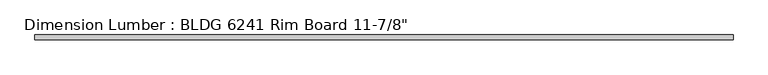
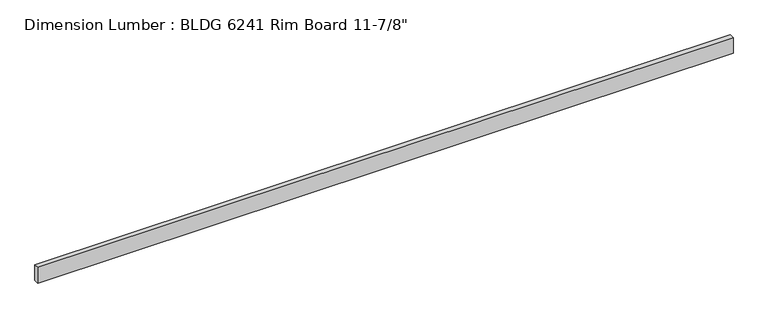
"""IFC4 building model written with IfcOpenShell, lengths in millimetres: beam geometry."""

import ifcopenshell
import ifcopenshell.guid

model = None  # the IFC model being written
_history = None  # IfcOwnerHistory: only IFC2X3 demands one
_inside = {}  # id of a spatial element -> (the spatial element, [elements in it])
_under = {}  # id of a project, library or spatial element -> (it, [spatial elements below it])
_declared = {}  # id of a project -> (the project, [libraries it declares])
_typed = {}  # id of a type object -> (the type object, [elements of that type])
_made_of = {}  # id of a material, layer set ... -> (it, [elements and type objects made of it])


def new_model(schema):
    """Start an empty IFC model of exactly this schema.

    Asked for "IFC4X3", IfcOpenShell would pick the latest addendum, in which some entities
    have other attributes; the version numbers below select the first issue.
    IFC2X3 requires an IfcOwnerHistory on every rooted entity: one is made here for all.
    """
    global model, _history
    if schema == "IFC4X3":
        model = ifcopenshell.file(schema_version=(4, 3, 0, 0))
    else:
        model = ifcopenshell.file(schema=schema)
    _inside.clear()
    _under.clear()
    _declared.clear()
    _typed.clear()
    _made_of.clear()
    _history = None
    if model.schema == "IFC2X3":
        org = make("IfcOrganization", Name="unknown")
        user = make(
            "IfcPersonAndOrganization",
            ThePerson=make("IfcPerson", FamilyName="unknown"),
            TheOrganization=org,
        )
        app = make(
            "IfcApplication",
            ApplicationDeveloper=org,
            Version="unknown",
            ApplicationFullName="unknown",
            ApplicationIdentifier="unknown",
        )
        _history = make(
            "IfcOwnerHistory",
            OwningUser=user,
            OwningApplication=app,
            ChangeAction="ADDED",
            CreationDate=0,
        )
    return model


def make(cls, **values):
    """One entity of the class cls with the attributes given. An attribute that is None is left unset."""
    return model.create_entity(
        cls, **{name: value for name, value in values.items() if value is not None}
    )


def rooted(cls, **values):
    """An entity with a GlobalId (a new one), such as an element, a storey or a relation."""
    return make(cls, GlobalId=ifcopenshell.guid.new(), OwnerHistory=_history, **values)


def si_unit(unit_type, name, prefix=None):
    """IfcSIUnit, for example si_unit("LENGTHUNIT", "METRE", prefix="MILLI")."""
    return make("IfcSIUnit", UnitType=unit_type, Prefix=prefix, Name=name)


def assignment(units):
    """IfcUnitAssignment: the units of a project."""
    return None if units is None else make("IfcUnitAssignment", Units=units)


def point(xyz):
    """IfcCartesianPoint."""
    return None if xyz is None else make("IfcCartesianPoint", Coordinates=xyz)


def direction(xyz):
    """IfcDirection."""
    return None if xyz is None else make("IfcDirection", DirectionRatios=xyz)


def frame(location, z_axis=None, x_axis=None):
    """IfcAxis2Placement3D, a coordinate frame: its origin and axes. An axis left out is left unset."""
    return make(
        "IfcAxis2Placement3D",
        Location=point(location),
        Axis=direction(z_axis),
        RefDirection=direction(x_axis),
    )


def origin():
    """The frame at (0, 0, 0) with its axes left unset."""
    return frame((0.0, 0.0, 0.0))


def place(relative_to, where):
    """IfcLocalPlacement: puts the frame where relative to a parent placement (None: the world)."""
    return make(
        "IfcLocalPlacement", PlacementRelTo=relative_to, RelativePlacement=where
    )


def context(
    kind, dimensions, precision=None, world=None, true_north=None, identifier=None
):
    """IfcGeometricRepresentationContext, for example the 3D "Model" context."""
    return make(
        "IfcGeometricRepresentationContext",
        ContextIdentifier=identifier,
        ContextType=kind,
        CoordinateSpaceDimension=dimensions,
        Precision=precision,
        WorldCoordinateSystem=world,
        TrueNorth=true_north,
    )


def project(units=None, contexts=None):
    """IfcProject with its units and contexts."""
    return rooted(
        "IfcProject",
        Name="project",
        RepresentationContexts=contexts,
        UnitsInContext=assignment(units),
    )


def spatial(cls, under=None, at=None, **own):
    """A site, building, storey or space (cls), placed at a placement, below another one or the project."""
    s = rooted(cls, ObjectPlacement=at, **own)
    if under is not None:
        _under.setdefault(under.id(), (under, []))[1].append(s)
    return s


def polyline(points):
    """IfcPolyline through the points."""
    return make("IfcPolyline", Points=[point(p) for p in points])


def outline(outer, holes=None, kind="AREA"):
    """IfcArbitraryClosedProfileDef: a profile drawn as a closed curve; with holes, ...WithVoids."""
    if holes is None:
        return make("IfcArbitraryClosedProfileDef", ProfileType=kind, OuterCurve=outer)
    return make(
        "IfcArbitraryProfileDefWithVoids",
        ProfileType=kind,
        OuterCurve=outer,
        InnerCurves=holes,
    )


def extrude(swept, where, along, depth):
    """IfcExtrudedAreaSolid: the profile swept, set in the frame where, extruded along a direction by depth."""
    return make(
        "IfcExtrudedAreaSolid",
        SweptArea=swept,
        Position=where,
        ExtrudedDirection=direction(along),
        Depth=depth,
    )


def shape(context_of_items, identifier, shape_type, items):
    """IfcShapeRepresentation: the items that make up one representation, for example the "Body"."""
    return make(
        "IfcShapeRepresentation",
        ContextOfItems=context_of_items,
        RepresentationIdentifier=identifier,
        RepresentationType=shape_type,
        Items=items,
    )


def source(mapping_origin, context_of_items, identifier, shape_type, items):
    """IfcRepresentationMap: a shape defined once, which mapped items show again and again."""
    return make(
        "IfcRepresentationMap",
        MappingOrigin=mapping_origin,
        MappedRepresentation=shape(context_of_items, identifier, shape_type, items),
    )


def transform(
    local_origin,
    x_axis=None,
    y_axis=None,
    z_axis=None,
    scale=None,
    scale2=None,
    scale3=None,
    uniform=True,
):
    """IfcCartesianTransformationOperator3D, or its non-uniform kind. x_axis, y_axis, z_axis: its Axis1, 2, 3."""
    if uniform:
        return make(
            "IfcCartesianTransformationOperator3D",
            Axis1=direction(x_axis),
            Axis2=direction(y_axis),
            LocalOrigin=point(local_origin),
            Scale=scale,
            Axis3=direction(z_axis),
        )
    return make(
        "IfcCartesianTransformationOperator3DnonUniform",
        Axis1=direction(x_axis),
        Axis2=direction(y_axis),
        LocalOrigin=point(local_origin),
        Scale=scale,
        Axis3=direction(z_axis),
        Scale2=scale2,
        Scale3=scale3,
    )


def mapped(mapping_source, mapping_target):
    """IfcMappedItem: shows the shape of a source again, moved by a transform."""
    return make(
        "IfcMappedItem", MappingSource=mapping_source, MappingTarget=mapping_target
    )


def made_of(thing, what):
    """Note that an element or type object is made of a material, layer set ...; save() writes the relation."""
    if what is not None:
        _made_of.setdefault(what.id(), (what, []))[1].append(thing)
    return thing


def element(
    cls,
    number,
    at=None,
    inside=None,
    cuts=None,
    type_object=None,
    material=None,
    context=None,
    identifier="Body",
    shape_type=None,
    held_by="IfcProductDefinitionShape",
    body=None,
    shapes=None,
    **own,
):
    """One element of the class cls, such as IfcWall. Its Tag is "e" and its number.

    at: its placement. inside: the storey or other place that contains it. cuts: it is an
    opening in that element (IfcRelVoidsElement). A single representation is given by context,
    identifier, shape_type and body (its items); several are given by shapes. held_by: the class
    of the entity that holds the representations. save() writes the other relations.
    """
    e = rooted(cls, Tag="e%d" % number, ObjectPlacement=at, **own)
    if body is not None:
        shapes = [shape(context, identifier, shape_type, body)]
    if shapes is not None:
        e.Representation = make(held_by, Representations=shapes)
    if inside is not None:
        _inside.setdefault(inside.id(), (inside, []))[1].append(e)
    if cuts is not None:
        rooted(
            "IfcRelVoidsElement", RelatingBuildingElement=cuts, RelatedOpeningElement=e
        )
    if type_object is not None:
        _typed.setdefault(type_object.id(), (type_object, []))[1].append(e)
    return made_of(e, material)


def aggregate(whole, parts):
    """IfcRelAggregates: a whole, such as a stair, and the parts it consists of."""
    return rooted("IfcRelAggregates", RelatingObject=whole, RelatedObjects=parts)


def save(model, path):
    """Write the relations noted so far, then the file.

    IfcRelAggregates (storeys below a building ...), IfcRelContainedInSpatialStructure (elements
    in a storey), IfcRelDefinesByType, IfcRelAssociatesMaterial and IfcRelDeclares: one each for
    every whole, place, type object, material and project.
    """
    for whole, parts in _under.values():
        aggregate(whole, parts)
    for where, things in _inside.values():
        rooted(
            "IfcRelContainedInSpatialStructure",
            RelatedElements=things,
            RelatingStructure=where,
        )
    for kind, things in _typed.values():
        rooted("IfcRelDefinesByType", RelatedObjects=things, RelatingType=kind)
    for what, things in _made_of.values():
        rooted("IfcRelAssociatesMaterial", RelatedObjects=things, RelatingMaterial=what)
    for by, libraries in _declared.values():
        rooted("IfcRelDeclares", RelatingContext=by, RelatedDefinitions=libraries)
    model.write(path)


def beam_06e53553(model_context):
    return source(origin(), model_context, "Body", "SweptSolid", [
        extrude(outline(polyline([(6332.8098719, 44.45), (6332.8098719, -44.45), (-6377.2598719, -44.45), (-6377.2598719, 44.45), (6332.8098719, 44.45)])), frame((0.0, 0.0, -150.8125), z_axis=(0.0, 0.0, 1.0), x_axis=(1.0, 0.0, 0.0)), (0.0, 0.0, 1.0), 301.625),
    ])


if __name__ == "__main__":
    model = new_model("IFC4")
    model_context = context("Model", 3, world=origin())
    ifc_project = project(units=[si_unit("LENGTHUNIT", "METRE", prefix="MILLI")], contexts=[model_context])
    site = spatial("IfcSite", under=ifc_project)
    building = spatial("IfcBuilding", under=site)
    placement = place(None, origin())
    beam_shape = beam_06e53553(model_context)
    element("IfcBeam", 1, ObjectType="Dimension Lumber : BLDG 6241 Rim Board 11-7/8\"", at=placement, inside=building, context=model_context, shape_type="MappedRepresentation", body=[
        mapped(beam_shape, transform((0.0, 0.0, 0.0), x_axis=(1.0, 0.0, 0.0), y_axis=(0.0, 1.0, 0.0), z_axis=(0.0, 0.0, 1.0))),
    ])
    save(model, "model.ifc")

# Revit data of these elements
# Type "Dimension Lumber : BLDG 6241 Rim Board 11-7/8\""
#   Assembly Code = "B10"
#   A = 0.273472 SF
#   Length [instance default] = 5' - 0"
#   b = 0' - 3 1/2"
#   d = 0' - 11 7/8"
#   Structural Material [instance default] = Softwood, Lumber
# Element 1 (IfcBeam, "Dimension Lumber : BLDG 6241 Rim Board 11-7/8\"")
#   Materials on its faces: "Softwood, Lumber"
# Materials
#   "Softwood, Lumber": class "Wood", colour RGB 223 192 134, transparency 0, Description = "Pinus Echinata", Cost = 0
